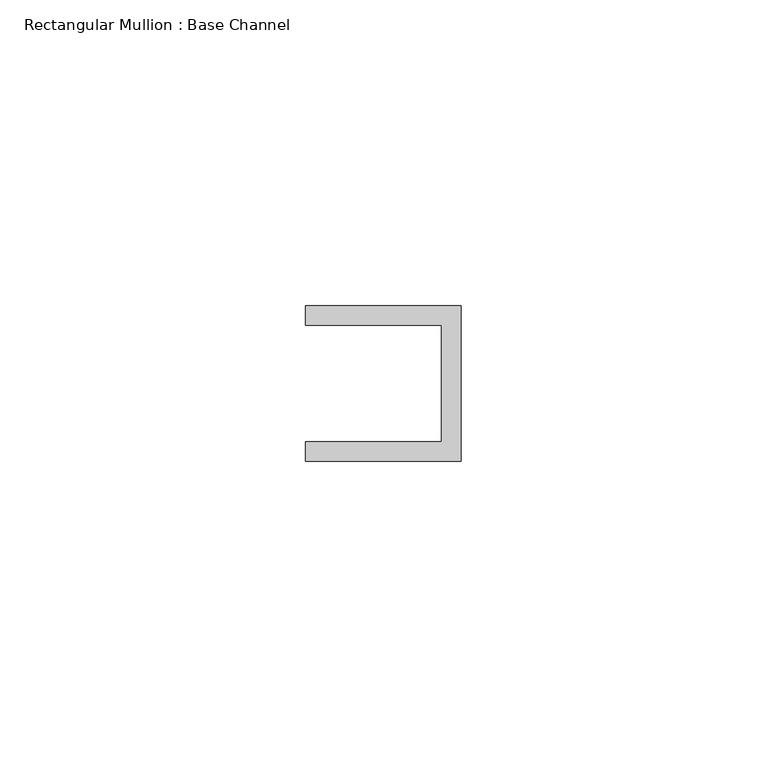
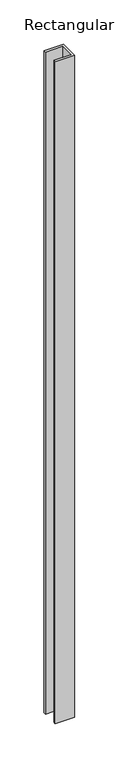
"""IFC4 building model written with IfcOpenShell, lengths in millimetres: member geometry, Rectangular Mullion : Base Channel."""

from ifc_helpers import new_model, si_unit, frame, origin, place, context, project, spatial, polyline, outline, extrude, source, transform, mapped, element, save


def rectangular_mullion_base_channel_648c15f3(model_context):
    return source(origin(), model_context, "Body", "SweptSolid", [
        extrude(outline(polyline([(0.0, -12.7), (-25.4, -12.7), (-25.4, -9.525), (-3.175, -9.525), (-3.175, 9.525), (-25.4, 9.525), (-25.4, 12.7), (0.0, 12.7), (0.0, -12.7)])), frame((0.0, 0.0, -914.3999999), z_axis=(0.0, 0.0, 1.0), x_axis=(1.0, 0.0, 0.0)), (0.0, 0.0, 1.0), 914.3999999),
    ])


if __name__ == "__main__":
    model = new_model("IFC4")
    model_context = context("Model", 3, world=origin())
    ifc_project = project(units=[si_unit("LENGTHUNIT", "METRE", prefix="MILLI")], contexts=[model_context])
    site = spatial("IfcSite", under=ifc_project)
    building = spatial("IfcBuilding", under=site)
    placement = place(None, origin())
    rectangular_mullion_base_channel_shape = rectangular_mullion_base_channel_648c15f3(model_context)
    element("IfcMember", 1, ObjectType="Rectangular Mullion : Base Channel", at=placement, inside=building, context=model_context, shape_type="MappedRepresentation", body=[
        mapped(rectangular_mullion_base_channel_shape, transform((0.0, 0.0, 0.0), x_axis=(1.0, 0.0, 0.0), y_axis=(0.0, 1.0, 0.0), z_axis=(0.0, 0.0, 1.0))),
    ])
    save(model, "model.ifc")

# Revit data of these elements
# Type "Rectangular Mullion : Base Channel"
#   built-in parameter 1007322 = 0.0833333 (stored number, unit not read)
#   built-in parameter 1007321 = 0.0416667 (stored number, unit not read)
#   built-in parameter 1007320 = -0.03125 (stored number, unit not read)
# Element 1 (IfcMember, "Rectangular Mullion : Base Channel")
#   Materials on its faces: "ALUM"
# Materials
#   "ALUM": class "Generic", colour RGB 157 157 157, transparency 0, Cost = 0
